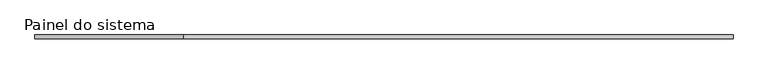
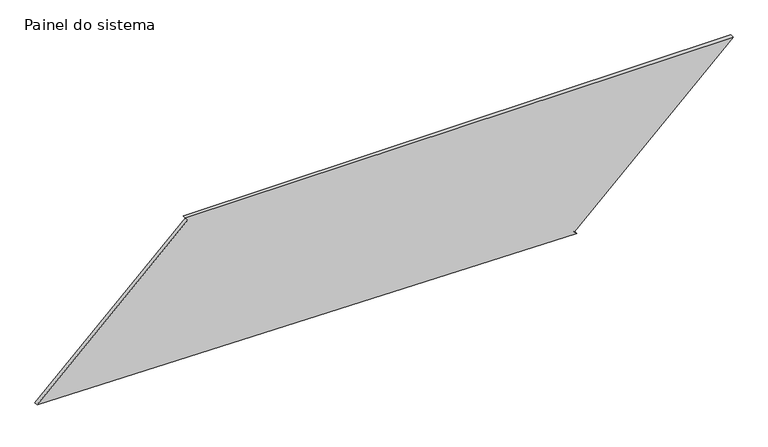
"""IFC4 building model written with IfcOpenShell, lengths in millimetres: plate geometry, Painel do sistema : Envidraçado."""

from ifc_helpers import new_model, si_unit, frame, origin, place, context, project, spatial, polyline, outline, extrude, source, transform, mapped, element, save


def painel_do_sistema_a6b5edca(model_context):
    return source(origin(), model_context, "Body", "SweptSolid", [
        extrude(outline(polyline([(0.0, 1296.6677439), (18.146416, 1279.4715935), (1036.0995907, 2353.6772355), (1036.0995907, -1350.1007665), (1017.9531747, -1332.9046162), (50.6349184, -2353.6772355), (0.0, 1296.6677439)])), frame((0.0, 24.5, 0.0), z_axis=(0.0, 1.0, 0.0), x_axis=(0.0, 0.0, 1.0)), (0.0, 0.0, 1.0), 25.0),
    ])


if __name__ == "__main__":
    model = new_model("IFC4")
    model_context = context("Model", 3, world=origin())
    ifc_project = project(units=[si_unit("LENGTHUNIT", "METRE", prefix="MILLI")], contexts=[model_context])
    site = spatial("IfcSite", under=ifc_project)
    building = spatial("IfcBuilding", under=site)
    placement = place(None, origin())
    painel_do_sistema_shape = painel_do_sistema_a6b5edca(model_context)
    element("IfcPlate", 1, ObjectType="Painel do sistema : Envidraçado", at=placement, inside=building, context=model_context, shape_type="MappedRepresentation", body=[
        mapped(painel_do_sistema_shape, transform((0.0, 0.0, 0.0), x_axis=(1.0, 0.0, 0.0), y_axis=(0.0, 1.0, 0.0), z_axis=(0.0, 0.0, 1.0))),
    ])
    save(model, "model.ifc")

# Revit data of these elements
# Type "Painel do sistema : Envidraçado"
#   Construction Type Id = "GSP4R"
#   Analytic Construction = "Vidraça única Pilkington 1/8 pol"
#   Visual Light Transmittance = 0.9
#   Solar Heat Gain Coefficient = 0.86
#   Heat Transfer Coefficient (U) = 6.7069 W/(m²·K)
# Element 1 (IfcPlate, "Painel do sistema : Envidraçado")
#   Materials on its faces: "Vidro"
# Materials
#   "Vidro": class "Vidro", colour RGB 0 128 192, transparency 0.9, Description = "Vidro de sílica", Cost = 0
